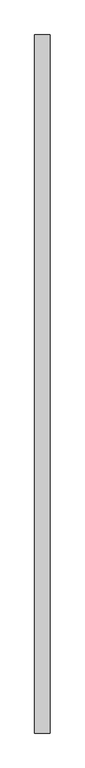
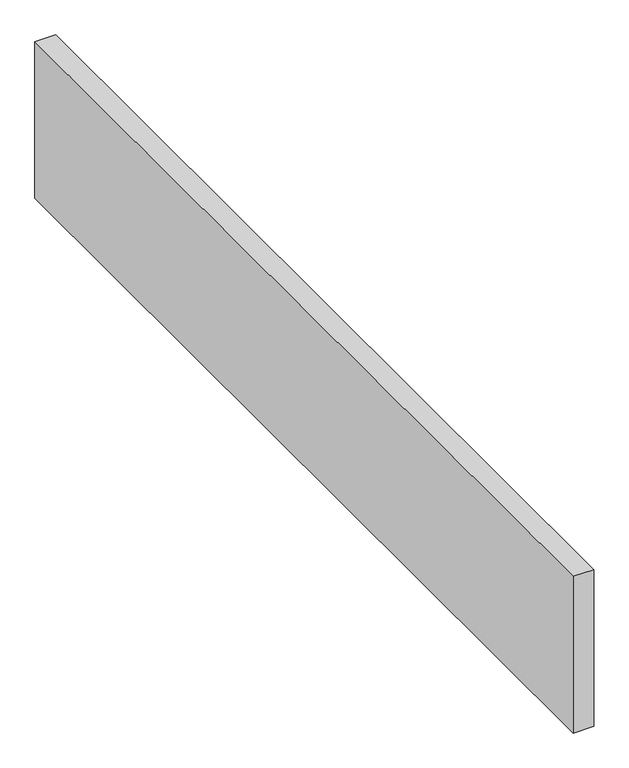
"""IFC4 building model written with IfcOpenShell, lengths in millimetres: proxy geometry, Framing045 416 : Framing045 416."""

from ifc_helpers import new_model, si_unit, frame, origin, place, context, project, spatial, polyline, outline, extrude, source, transform, mapped, element, save


def generic_models_23d6586b(model_context):
    return source(origin(), model_context, "Body", "SweptSolid", [
        extrude(outline(polyline([(-4972.599396, 7982.1531721), (-5017.049396, 7982.1531721), (-5017.049396, 9982.1531721), (-4972.599396, 9982.1531721), (-4972.599396, 7982.1531721)])), frame((0.0, 0.0, 43056.5101822), z_axis=(0.0, 0.0, 1.0), x_axis=(1.0, 0.0, 0.0)), (0.0, 0.0, 1.0), 355.2981173),
    ])


if __name__ == "__main__":
    model = new_model("IFC4")
    model_context = context("Model", 3, world=origin())
    ifc_project = project(units=[si_unit("LENGTHUNIT", "METRE", prefix="MILLI")], contexts=[model_context])
    site = spatial("IfcSite", under=ifc_project)
    building = spatial("IfcBuilding", under=site)
    placement = place(None, origin())
    generic_models_shape = generic_models_23d6586b(model_context)
    element("IfcBuildingElementProxy", 1, Name="Framing045 416 : Framing045 416", ObjectType="Framing045 416 : Framing045 416", at=placement, inside=building, context=model_context, shape_type="MappedRepresentation", body=[
        mapped(generic_models_shape, transform((0.0, 0.0, 0.0), x_axis=(1.0, 0.0, 0.0), y_axis=(0.0, 1.0, 0.0), z_axis=(0.0, 0.0, 1.0))),
    ])
    save(model, "model.ifc")

# Revit data of these elements
# Type "Framing045 416 : Framing045 416"
#   NameOverride = "Framing045"
# Element 1 (IfcBuildingElementProxy, "Framing045 416 : Framing045 416")
#   Materials on its faces: "WOOD FRAMING (SEE STRUCT DWGS)"
# Materials
#   "WOOD FRAMING (SEE STRUCT DWGS)": class "Unassigned", colour RGB 224 188 168, transparency 0, Cost = 0
